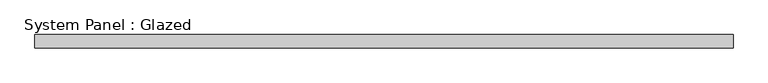
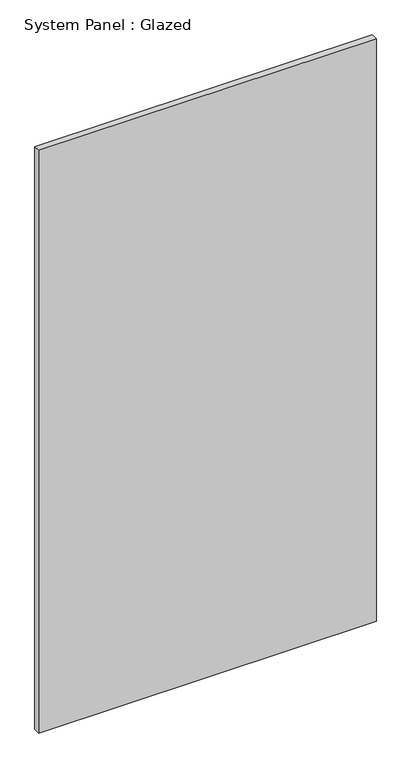
"""IFC4 building model written with IfcOpenShell, lengths in millimetres: plate geometry, System Panel : Glazed."""

import ifcopenshell
import ifcopenshell.guid

model = None  # the IFC model being written
_history = None  # IfcOwnerHistory: only IFC2X3 demands one
_inside = {}  # id of a spatial element -> (the spatial element, [elements in it])
_under = {}  # id of a project, library or spatial element -> (it, [spatial elements below it])
_declared = {}  # id of a project -> (the project, [libraries it declares])
_typed = {}  # id of a type object -> (the type object, [elements of that type])
_made_of = {}  # id of a material, layer set ... -> (it, [elements and type objects made of it])


def new_model(schema):
    """Start an empty IFC model of exactly this schema.

    Asked for "IFC4X3", IfcOpenShell would pick the latest addendum, in which some entities
    have other attributes; the version numbers below select the first issue.
    IFC2X3 requires an IfcOwnerHistory on every rooted entity: one is made here for all.
    """
    global model, _history
    if schema == "IFC4X3":
        model = ifcopenshell.file(schema_version=(4, 3, 0, 0))
    else:
        model = ifcopenshell.file(schema=schema)
    _inside.clear()
    _under.clear()
    _declared.clear()
    _typed.clear()
    _made_of.clear()
    _history = None
    if model.schema == "IFC2X3":
        org = make("IfcOrganization", Name="unknown")
        user = make(
            "IfcPersonAndOrganization",
            ThePerson=make("IfcPerson", FamilyName="unknown"),
            TheOrganization=org,
        )
        app = make(
            "IfcApplication",
            ApplicationDeveloper=org,
            Version="unknown",
            ApplicationFullName="unknown",
            ApplicationIdentifier="unknown",
        )
        _history = make(
            "IfcOwnerHistory",
            OwningUser=user,
            OwningApplication=app,
            ChangeAction="ADDED",
            CreationDate=0,
        )
    return model


def make(cls, **values):
    """One entity of the class cls with the attributes given. An attribute that is None is left unset."""
    return model.create_entity(
        cls, **{name: value for name, value in values.items() if value is not None}
    )


def rooted(cls, **values):
    """An entity with a GlobalId (a new one), such as an element, a storey or a relation."""
    return make(cls, GlobalId=ifcopenshell.guid.new(), OwnerHistory=_history, **values)


def si_unit(unit_type, name, prefix=None):
    """IfcSIUnit, for example si_unit("LENGTHUNIT", "METRE", prefix="MILLI")."""
    return make("IfcSIUnit", UnitType=unit_type, Prefix=prefix, Name=name)


def assignment(units):
    """IfcUnitAssignment: the units of a project."""
    return None if units is None else make("IfcUnitAssignment", Units=units)


def point(xyz):
    """IfcCartesianPoint."""
    return None if xyz is None else make("IfcCartesianPoint", Coordinates=xyz)


def direction(xyz):
    """IfcDirection."""
    return None if xyz is None else make("IfcDirection", DirectionRatios=xyz)


def frame(location, z_axis=None, x_axis=None):
    """IfcAxis2Placement3D, a coordinate frame: its origin and axes. An axis left out is left unset."""
    return make(
        "IfcAxis2Placement3D",
        Location=point(location),
        Axis=direction(z_axis),
        RefDirection=direction(x_axis),
    )


def origin():
    """The frame at (0, 0, 0) with its axes left unset."""
    return frame((0.0, 0.0, 0.0))


def origin_with_axes():
    """The frame at (0, 0, 0) with the z axis (0, 0, 1) and the x axis (1, 0, 0) written out."""
    return frame((0.0, 0.0, 0.0), z_axis=(0.0, 0.0, 1.0), x_axis=(1.0, 0.0, 0.0))


def place(relative_to, where):
    """IfcLocalPlacement: puts the frame where relative to a parent placement (None: the world)."""
    return make(
        "IfcLocalPlacement", PlacementRelTo=relative_to, RelativePlacement=where
    )


def context(
    kind, dimensions, precision=None, world=None, true_north=None, identifier=None
):
    """IfcGeometricRepresentationContext, for example the 3D "Model" context."""
    return make(
        "IfcGeometricRepresentationContext",
        ContextIdentifier=identifier,
        ContextType=kind,
        CoordinateSpaceDimension=dimensions,
        Precision=precision,
        WorldCoordinateSystem=world,
        TrueNorth=true_north,
    )


def project(units=None, contexts=None):
    """IfcProject with its units and contexts."""
    return rooted(
        "IfcProject",
        Name="project",
        RepresentationContexts=contexts,
        UnitsInContext=assignment(units),
    )


def spatial(cls, under=None, at=None, **own):
    """A site, building, storey or space (cls), placed at a placement, below another one or the project."""
    s = rooted(cls, ObjectPlacement=at, **own)
    if under is not None:
        _under.setdefault(under.id(), (under, []))[1].append(s)
    return s


def polyline(points):
    """IfcPolyline through the points."""
    return make("IfcPolyline", Points=[point(p) for p in points])


def outline(outer, holes=None, kind="AREA"):
    """IfcArbitraryClosedProfileDef: a profile drawn as a closed curve; with holes, ...WithVoids."""
    if holes is None:
        return make("IfcArbitraryClosedProfileDef", ProfileType=kind, OuterCurve=outer)
    return make(
        "IfcArbitraryProfileDefWithVoids",
        ProfileType=kind,
        OuterCurve=outer,
        InnerCurves=holes,
    )


def extrude(swept, where, along, depth):
    """IfcExtrudedAreaSolid: the profile swept, set in the frame where, extruded along a direction by depth."""
    return make(
        "IfcExtrudedAreaSolid",
        SweptArea=swept,
        Position=where,
        ExtrudedDirection=direction(along),
        Depth=depth,
    )


def shape(context_of_items, identifier, shape_type, items):
    """IfcShapeRepresentation: the items that make up one representation, for example the "Body"."""
    return make(
        "IfcShapeRepresentation",
        ContextOfItems=context_of_items,
        RepresentationIdentifier=identifier,
        RepresentationType=shape_type,
        Items=items,
    )


def source(mapping_origin, context_of_items, identifier, shape_type, items):
    """IfcRepresentationMap: a shape defined once, which mapped items show again and again."""
    return make(
        "IfcRepresentationMap",
        MappingOrigin=mapping_origin,
        MappedRepresentation=shape(context_of_items, identifier, shape_type, items),
    )


def transform(
    local_origin,
    x_axis=None,
    y_axis=None,
    z_axis=None,
    scale=None,
    scale2=None,
    scale3=None,
    uniform=True,
):
    """IfcCartesianTransformationOperator3D, or its non-uniform kind. x_axis, y_axis, z_axis: its Axis1, 2, 3."""
    if uniform:
        return make(
            "IfcCartesianTransformationOperator3D",
            Axis1=direction(x_axis),
            Axis2=direction(y_axis),
            LocalOrigin=point(local_origin),
            Scale=scale,
            Axis3=direction(z_axis),
        )
    return make(
        "IfcCartesianTransformationOperator3DnonUniform",
        Axis1=direction(x_axis),
        Axis2=direction(y_axis),
        LocalOrigin=point(local_origin),
        Scale=scale,
        Axis3=direction(z_axis),
        Scale2=scale2,
        Scale3=scale3,
    )


def mapped(mapping_source, mapping_target):
    """IfcMappedItem: shows the shape of a source again, moved by a transform."""
    return make(
        "IfcMappedItem", MappingSource=mapping_source, MappingTarget=mapping_target
    )


def made_of(thing, what):
    """Note that an element or type object is made of a material, layer set ...; save() writes the relation."""
    if what is not None:
        _made_of.setdefault(what.id(), (what, []))[1].append(thing)
    return thing


def element(
    cls,
    number,
    at=None,
    inside=None,
    cuts=None,
    type_object=None,
    material=None,
    context=None,
    identifier="Body",
    shape_type=None,
    held_by="IfcProductDefinitionShape",
    body=None,
    shapes=None,
    **own,
):
    """One element of the class cls, such as IfcWall. Its Tag is "e" and its number.

    at: its placement. inside: the storey or other place that contains it. cuts: it is an
    opening in that element (IfcRelVoidsElement). A single representation is given by context,
    identifier, shape_type and body (its items); several are given by shapes. held_by: the class
    of the entity that holds the representations. save() writes the other relations.
    """
    e = rooted(cls, Tag="e%d" % number, ObjectPlacement=at, **own)
    if body is not None:
        shapes = [shape(context, identifier, shape_type, body)]
    if shapes is not None:
        e.Representation = make(held_by, Representations=shapes)
    if inside is not None:
        _inside.setdefault(inside.id(), (inside, []))[1].append(e)
    if cuts is not None:
        rooted(
            "IfcRelVoidsElement", RelatingBuildingElement=cuts, RelatedOpeningElement=e
        )
    if type_object is not None:
        _typed.setdefault(type_object.id(), (type_object, []))[1].append(e)
    return made_of(e, material)


def aggregate(whole, parts):
    """IfcRelAggregates: a whole, such as a stair, and the parts it consists of."""
    return rooted("IfcRelAggregates", RelatingObject=whole, RelatedObjects=parts)


def save(model, path):
    """Write the relations noted so far, then the file.

    IfcRelAggregates (storeys below a building ...), IfcRelContainedInSpatialStructure (elements
    in a storey), IfcRelDefinesByType, IfcRelAssociatesMaterial and IfcRelDeclares: one each for
    every whole, place, type object, material and project.
    """
    for whole, parts in _under.values():
        aggregate(whole, parts)
    for where, things in _inside.values():
        rooted(
            "IfcRelContainedInSpatialStructure",
            RelatedElements=things,
            RelatingStructure=where,
        )
    for kind, things in _typed.values():
        rooted("IfcRelDefinesByType", RelatedObjects=things, RelatingType=kind)
    for what, things in _made_of.values():
        rooted("IfcRelAssociatesMaterial", RelatedObjects=things, RelatingMaterial=what)
    for by, libraries in _declared.values():
        rooted("IfcRelDeclares", RelatingContext=by, RelatedDefinitions=libraries)
    model.write(path)


def system_panel_glazed_9c6a85c7(model_context):
    return source(origin(), model_context, "Body", "SweptSolid", [
        extrude(outline(polyline([(658.3333334, 24.5), (-658.3333334, 24.5), (-658.3333334, 49.5), (658.3333334, 49.5), (658.3333334, 24.5)])), origin_with_axes(), (0.0, 0.0, 1.0), 2400.0),
    ])


if __name__ == "__main__":
    model = new_model("IFC4")
    model_context = context("Model", 3, world=origin())
    ifc_project = project(units=[si_unit("LENGTHUNIT", "METRE", prefix="MILLI")], contexts=[model_context])
    site = spatial("IfcSite", under=ifc_project)
    building = spatial("IfcBuilding", under=site)
    placement = place(None, origin())
    system_panel_glazed_shape = system_panel_glazed_9c6a85c7(model_context)
    element("IfcPlate", 1, ObjectType="System Panel : Glazed", at=placement, inside=building, context=model_context, shape_type="MappedRepresentation", body=[
        mapped(system_panel_glazed_shape, transform((0.0, 0.0, 0.0), x_axis=(1.0, 0.0, 0.0), y_axis=(0.0, 1.0, 0.0), z_axis=(0.0, 0.0, 1.0))),
    ])
    save(model, "model.ifc")

# Revit data of these elements
# Type "System Panel : Glazed"
#   Keynote = "H11"
#   Construction Type Id = "GSP4R"
#   Analytic Construction = "1/8 in Pilkington single glazing"
#   Visual Light Transmittance = 0.9
#   Solar Heat Gain Coefficient = 0.86
#   Heat Transfer Coefficient (U) = 6.7069 W/(m²·K)
#   Define Thermal Properties by = 1
# Element 1 (IfcPlate, "System Panel : Glazed")
#   Materials on its faces: "Glass"
# Materials
#   "Glass": class "Glass", colour RGB 0 128 192, transparency 0.9, Description = "Soda Lime Glass", Cost = 0
